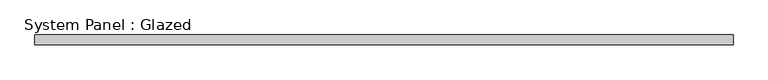
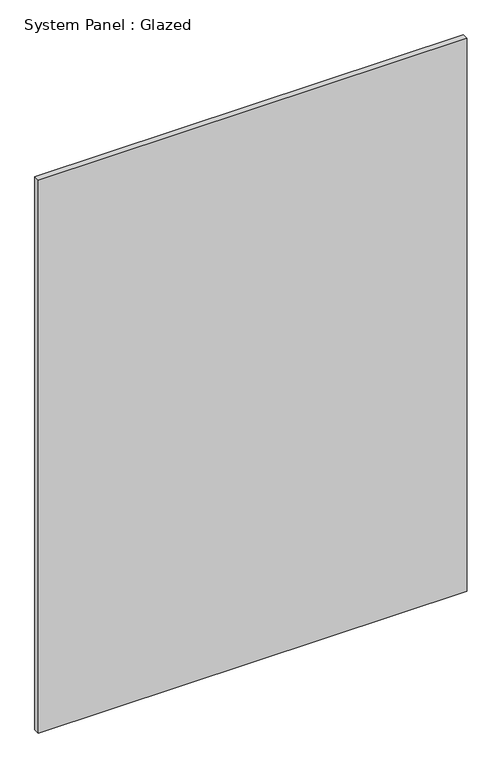
"""IFC4 building model written with IfcOpenShell, lengths in millimetres: plate geometry, System Panel : Glazed."""

from ifc_helpers import new_model, si_unit, origin, origin_with_axes, place, context, project, spatial, polyline, outline, extrude, source, transform, mapped, element, save


def system_panel_glazed_37b58b52(model_context):
    return source(origin(), model_context, "Body", "SweptSolid", [
        extrude(outline(polyline([(890.0, 24.5), (-890.0, 24.5), (-890.0, 49.5), (890.0, 49.5), (890.0, 24.5)])), origin_with_axes(), (0.0, 0.0, 1.0), 2425.0),
    ])


if __name__ == "__main__":
    model = new_model("IFC4")
    model_context = context("Model", 3, world=origin())
    ifc_project = project(units=[si_unit("LENGTHUNIT", "METRE", prefix="MILLI")], contexts=[model_context])
    site = spatial("IfcSite", under=ifc_project)
    building = spatial("IfcBuilding", under=site)
    placement = place(None, origin())
    system_panel_glazed_shape = system_panel_glazed_37b58b52(model_context)
    element("IfcPlate", 1, ObjectType="System Panel : Glazed", at=placement, inside=building, context=model_context, shape_type="MappedRepresentation", body=[
        mapped(system_panel_glazed_shape, transform((0.0, 0.0, 0.0), x_axis=(1.0, 0.0, 0.0), y_axis=(0.0, 1.0, 0.0), z_axis=(0.0, 0.0, 1.0))),
    ])
    save(model, "model.ifc")

# Revit data of these elements
# Type "System Panel : Glazed"
#   Keynote = "H11"
#   Construction Type Id = "GSP4R"
#   Analytic Construction = "1/8 in Pilkington single glazing"
#   Visual Light Transmittance = 0.9
#   Solar Heat Gain Coefficient = 0.86
#   Heat Transfer Coefficient (U) = 6.7069 W/(m²·K)
# Element 1 (IfcPlate, "System Panel : Glazed")
#   Materials on its faces: "Glass"
# Materials
#   "Glass": class "Glass", colour RGB 0 128 192, transparency 0.9, Description = "Soda Lime Glass", Cost = 0
